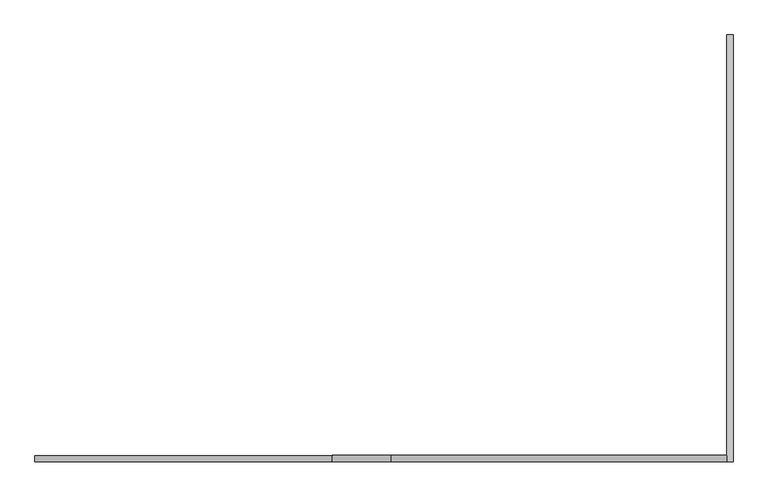
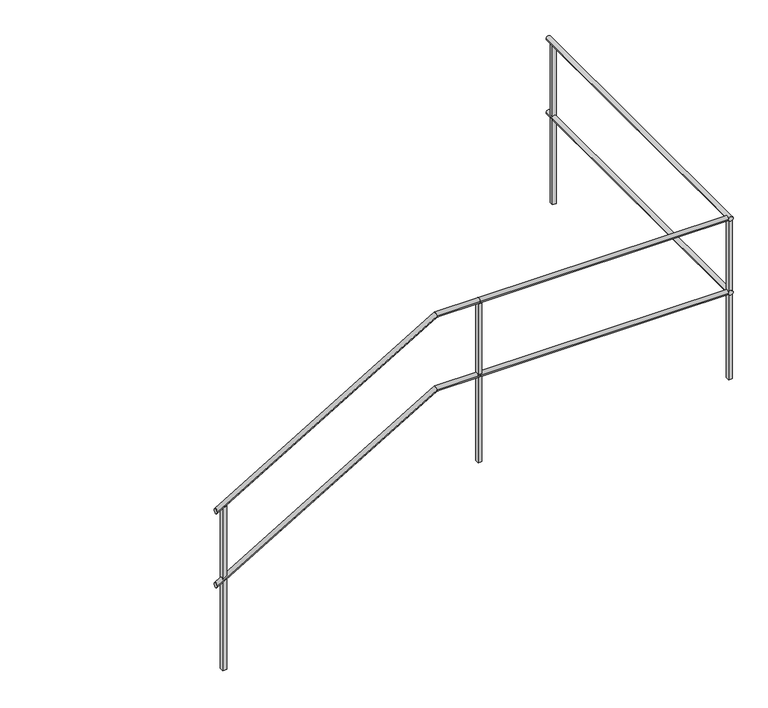
"""IFC4 building model written with IfcOpenShell, lengths in millimetres: railing geometry."""

from ifc_helpers import new_model, si_unit, frame, origin, place, context, project, spatial, polyline, circle_curve, ellipse_curve, outline, extrude, source, transform, mapped, element, save
from ifc_brep_helpers import plane_surface, cylinder_surface, advanced_brep


def railing_42641741(model_context):
    return source(origin(), model_context, "Body", "SolidModel", [
        advanced_brep(
        [(35195.0, -1335.0791411, 749.1723166), (35195.0, -1365.0791411, 749.1723166), (36599.1264386, -1335.0791411, 1584.9618634), (36599.1264386, -1365.0791411, 1584.9618634), (36875.0, -1335.0791411, 1584.9618634), (36875.0, -1365.0791411, 1584.9618634)],
        [
            (0, 1, ellipse_curve(frame((35195.0, -1350.0791411, 749.1723166), z_axis=(-1.0, 0.0, 0.0), x_axis=(0.0, 0.0, -1.0)), 17.4562134, 15.0)),
            (1, 0, ellipse_curve(frame((35195.0, -1350.0791411, 749.1723166), z_axis=(-1.0, 0.0, 0.0), x_axis=(0.0, 0.0, -1.0)), 17.4562134, 15.0)),
            (0, 2),
            (2, 3, ellipse_curve(frame((36599.1264386, -1350.0791411, 1584.9618634), z_axis=(-0.9641817474962143, 0.0, -0.265242450967311), x_axis=(0.265242450967311, 0.0, -0.9641817474962145)), 15.5572329, 15.0)),
            (3, 1),
            (3, 2, ellipse_curve(frame((36599.1264386, -1350.0791411, 1584.9618634), z_axis=(-0.9641817474962143, 0.0, -0.265242450967311), x_axis=(0.265242450967311, 0.0, -0.9641817474962145)), 15.5572329, 15.0)),
            (4, 5, circle_curve(frame((36875.0, -1350.0791411, 1584.9618634), z_axis=(1.0, 0.0, 0.0), x_axis=(0.0, -1.0, 0.0)), 15.0)),
            (5, 4, circle_curve(frame((36875.0, -1350.0791411, 1584.9618634), z_axis=(1.0, 0.0, 0.0), x_axis=(0.0, -1.0, 0.0)), 15.0)),
            (2, 4),
            (5, 3),
        ],
        [
            plane_surface(frame((35195.0, -1350.0791411, 766.62853), z_axis=(-1.0, 0.0, 0.0), x_axis=(0.0, 1.0, 0.0))),
            cylinder_surface(frame((35202.6722579, -1350.0791411, 753.7391368), z_axis=(-0.8592928844097072, 0.0, -0.5114838597676818), x_axis=(0.0, -1.0, 0.0)), 15.0),
            plane_surface(frame((36875.0, -1350.0791411, 1599.9618634), z_axis=(1.0, 0.0, 0.0), x_axis=(0.0, 1.0, 0.0))),
            cylinder_surface(frame((36595.0, -1350.0791411, 1584.9618634), z_axis=(-1.0, 0.0, 0.0), x_axis=(0.0, -1.0, 0.0)), 15.0),
        ],
        [
            (0, [[1, 2]]),
            (1, [[-1, 3, 4, 5]]),
            (1, [[-2, -5, 6, -3]]),
            (2, [[7, 8]]),
            (3, [[-4, 9, -8, 10]]),
            (3, [[-6, -10, -7, -9]]),
        ],
    ),
        advanced_brep(
        [(36875.0, -1335.0791411, 1584.9618634), (36875.0, -1365.0791411, 1584.9618634), (38459.6, -1335.0791411, 1584.9618634), (38459.6, -1365.0791411, 1584.9618634)],
        [
            (0, 1, circle_curve(frame((36875.0, -1350.0791411, 1584.9618634), z_axis=(-1.0, 0.0, 0.0), x_axis=(0.0, -1.0, 0.0)), 15.0)),
            (1, 0, circle_curve(frame((36875.0, -1350.0791411, 1584.9618634), z_axis=(-1.0, 0.0, 0.0), x_axis=(0.0, -1.0, 0.0)), 15.0)),
            (2, 3, circle_curve(frame((38459.6, -1350.0791411, 1584.9618634), z_axis=(1.0, 0.0, 0.0), x_axis=(0.0, -1.0, 0.0)), 15.0)),
            (3, 2, circle_curve(frame((38459.6, -1350.0791411, 1584.9618634), z_axis=(1.0, 0.0, 0.0), x_axis=(0.0, -1.0, 0.0)), 15.0)),
            (0, 2),
            (3, 1),
        ],
        [
            plane_surface(frame((36875.0, -1350.0791411, 1599.9618634), z_axis=(-1.0, 0.0, 0.0), x_axis=(0.0, 1.0, 0.0))),
            plane_surface(frame((38459.6, -1350.0791411, 1599.9618634), z_axis=(1.0, 0.0, 0.0), x_axis=(0.0, 1.0, 0.0))),
            cylinder_surface(frame((36875.0, -1350.0791411, 1584.9618634), z_axis=(-1.0, 0.0, 0.0), x_axis=(0.0, -1.0, 0.0)), 15.0),
        ],
        [
            (0, [[1, 2]]),
            (1, [[3, 4]]),
            (2, [[-1, 5, -4, 6]]),
            (2, [[-2, -6, -3, -5]]),
        ],
    ),
        advanced_brep(
        [(38459.6, -1365.0791411, 1584.9618634), (38489.6, -1365.0791411, 1584.9618634), (38459.6, 649.5208589, 1584.9618634), (38489.6, 649.5208589, 1584.9618634)],
        [
            (0, 1, circle_curve(frame((38474.6, -1365.0791411, 1584.9618634), z_axis=(0.0, -1.0, 0.0), x_axis=(1.0, 0.0, 0.0)), 15.0)),
            (1, 0, circle_curve(frame((38474.6, -1365.0791411, 1584.9618634), z_axis=(0.0, -1.0, 0.0), x_axis=(1.0, 0.0, 0.0)), 15.0)),
            (2, 3, circle_curve(frame((38474.6, 649.5208589, 1584.9618634), z_axis=(0.0, 1.0, 0.0), x_axis=(1.0, 0.0, 0.0)), 15.0)),
            (3, 2, circle_curve(frame((38474.6, 649.5208589, 1584.9618634), z_axis=(0.0, 1.0, 0.0), x_axis=(1.0, 0.0, 0.0)), 15.0)),
            (0, 2),
            (3, 1),
        ],
        [
            plane_surface(frame((38474.6, -1365.0791411, 1599.9618634), z_axis=(0.0, -1.0, 0.0), x_axis=(0.0, 0.0, 1.0))),
            plane_surface(frame((38474.6, 649.5208589, 1599.9618634), z_axis=(0.0, 1.0, 0.0), x_axis=(0.0, 0.0, 1.0))),
            cylinder_surface(frame((38474.6, -1365.0791411, 1584.9618634), z_axis=(0.0, -1.0, 0.0), x_axis=(1.0, 0.0, 0.0)), 15.0),
        ],
        [
            (0, [[1, 2]]),
            (1, [[3, 4]]),
            (2, [[-1, 5, -4, 6]]),
            (2, [[-2, -6, -3, -5]]),
        ],
    ),
        advanced_brep(
        [(35195.0, -1335.0791411, 1249.1723166), (35195.0, -1365.0791411, 1249.1723166), (36599.1264386, -1335.0791411, 2084.9618634), (36599.1264386, -1365.0791411, 2084.9618634), (36875.0, -1335.0791411, 2084.9618634), (36875.0, -1365.0791411, 2084.9618634)],
        [
            (0, 1, ellipse_curve(frame((35195.0, -1350.0791411, 1249.1723166), z_axis=(-1.0, 0.0, 0.0), x_axis=(0.0, 0.0, -1.0)), 17.4562134, 15.0)),
            (1, 0, ellipse_curve(frame((35195.0, -1350.0791411, 1249.1723166), z_axis=(-1.0, 0.0, 0.0), x_axis=(0.0, 0.0, -1.0)), 17.4562134, 15.0)),
            (0, 2),
            (2, 3, ellipse_curve(frame((36599.1264386, -1350.0791411, 2084.9618634), z_axis=(-0.9641817474962143, 0.0, -0.265242450967311), x_axis=(0.265242450967311, 0.0, -0.9641817474962145)), 15.5572329, 15.0)),
            (3, 1),
            (3, 2, ellipse_curve(frame((36599.1264386, -1350.0791411, 2084.9618634), z_axis=(-0.9641817474962143, 0.0, -0.265242450967311), x_axis=(0.265242450967311, 0.0, -0.9641817474962145)), 15.5572329, 15.0)),
            (4, 5, circle_curve(frame((36875.0, -1350.0791411, 2084.9618634), z_axis=(1.0, 0.0, 0.0), x_axis=(0.0, -1.0, 0.0)), 15.0)),
            (5, 4, circle_curve(frame((36875.0, -1350.0791411, 2084.9618634), z_axis=(1.0, 0.0, 0.0), x_axis=(0.0, -1.0, 0.0)), 15.0)),
            (2, 4),
            (5, 3),
        ],
        [
            plane_surface(frame((35195.0, -1350.0791411, 1266.62853), z_axis=(-1.0, 0.0, 0.0), x_axis=(0.0, 1.0, 0.0))),
            cylinder_surface(frame((35202.6722579, -1350.0791411, 1253.7391368), z_axis=(-0.8592928844097072, 0.0, -0.5114838597676818), x_axis=(0.0, -1.0, 0.0)), 15.0),
            plane_surface(frame((36875.0, -1350.0791411, 2099.9618634), z_axis=(1.0, 0.0, 0.0), x_axis=(0.0, 1.0, 0.0))),
            cylinder_surface(frame((36595.0, -1350.0791411, 2084.9618634), z_axis=(-1.0, 0.0, 0.0), x_axis=(0.0, -1.0, 0.0)), 15.0),
        ],
        [
            (0, [[1, 2]]),
            (1, [[-1, 3, 4, 5]]),
            (1, [[-2, -5, 6, -3]]),
            (2, [[7, 8]]),
            (3, [[-4, 9, -8, 10]]),
            (3, [[-6, -10, -7, -9]]),
        ],
    ),
        advanced_brep(
        [(36875.0, -1335.0791411, 2084.9618634), (36875.0, -1365.0791411, 2084.9618634), (38459.6, -1335.0791411, 2084.9618634), (38459.6, -1365.0791411, 2084.9618634)],
        [
            (0, 1, circle_curve(frame((36875.0, -1350.0791411, 2084.9618634), z_axis=(-1.0, 0.0, 0.0), x_axis=(0.0, -1.0, 0.0)), 15.0)),
            (1, 0, circle_curve(frame((36875.0, -1350.0791411, 2084.9618634), z_axis=(-1.0, 0.0, 0.0), x_axis=(0.0, -1.0, 0.0)), 15.0)),
            (2, 3, circle_curve(frame((38459.6, -1350.0791411, 2084.9618634), z_axis=(1.0, 0.0, 0.0), x_axis=(0.0, -1.0, 0.0)), 15.0)),
            (3, 2, circle_curve(frame((38459.6, -1350.0791411, 2084.9618634), z_axis=(1.0, 0.0, 0.0), x_axis=(0.0, -1.0, 0.0)), 15.0)),
            (0, 2),
            (3, 1),
        ],
        [
            plane_surface(frame((36875.0, -1350.0791411, 2099.9618634), z_axis=(-1.0, 0.0, 0.0), x_axis=(0.0, 1.0, 0.0))),
            plane_surface(frame((38459.6, -1350.0791411, 2099.9618634), z_axis=(1.0, 0.0, 0.0), x_axis=(0.0, 1.0, 0.0))),
            cylinder_surface(frame((36875.0, -1350.0791411, 2084.9618634), z_axis=(-1.0, 0.0, 0.0), x_axis=(0.0, -1.0, 0.0)), 15.0),
        ],
        [
            (0, [[1, 2]]),
            (1, [[3, 4]]),
            (2, [[-1, 5, -4, 6]]),
            (2, [[-2, -6, -3, -5]]),
        ],
    ),
        advanced_brep(
        [(38459.6, -1365.0791411, 2084.9618634), (38489.6, -1365.0791411, 2084.9618634), (38459.6, 649.5208589, 2084.9618634), (38489.6, 649.5208589, 2084.9618634)],
        [
            (0, 1, circle_curve(frame((38474.6, -1365.0791411, 2084.9618634), z_axis=(0.0, -1.0, 0.0), x_axis=(1.0, 0.0, 0.0)), 15.0)),
            (1, 0, circle_curve(frame((38474.6, -1365.0791411, 2084.9618634), z_axis=(0.0, -1.0, 0.0), x_axis=(1.0, 0.0, 0.0)), 15.0)),
            (2, 3, circle_curve(frame((38474.6, 649.5208589, 2084.9618634), z_axis=(0.0, 1.0, 0.0), x_axis=(1.0, 0.0, 0.0)), 15.0)),
            (3, 2, circle_curve(frame((38474.6, 649.5208589, 2084.9618634), z_axis=(0.0, 1.0, 0.0), x_axis=(1.0, 0.0, 0.0)), 15.0)),
            (0, 2),
            (3, 1),
        ],
        [
            plane_surface(frame((38474.6, -1365.0791411, 2099.9618634), z_axis=(0.0, -1.0, 0.0), x_axis=(0.0, 0.0, 1.0))),
            plane_surface(frame((38474.6, 649.5208589, 2099.9618634), z_axis=(0.0, 1.0, 0.0), x_axis=(0.0, 0.0, 1.0))),
            cylinder_surface(frame((38474.6, -1365.0791411, 2084.9618634), z_axis=(0.0, -1.0, 0.0), x_axis=(1.0, 0.0, 0.0)), 15.0),
        ],
        [
            (0, [[1, 2]]),
            (1, [[3, 4]]),
            (2, [[-1, 5, -4, 6]]),
            (2, [[-2, -6, -3, -5]]),
        ],
    ),
        extrude(outline(polyline([(38462.1, -1362.5791411), (38462.1, -1337.5791411), (38487.1, -1337.5791411), (38487.1, -1362.5791411), (38462.1, -1362.5791411)])), frame((0.0, 0.0, 999.9618634), z_axis=(0.0, 0.0, 1.0), x_axis=(1.0, 0.0, 0.0)), (0.0, 0.0, 1.0), 1070.0),
        extrude(outline(polyline([(36862.5, -1362.5791411), (36862.5, -1337.5791411), (36887.5, -1337.5791411), (36887.5, -1362.5791411), (36862.5, -1362.5791411)])), frame((0.0, 0.0, 999.9618634), z_axis=(0.0, 0.0, 1.0), x_axis=(1.0, 0.0, 0.0)), (0.0, 0.0, 1.0), 1070.0),
        extrude(outline(polyline([(38487.1, 587.0208589), (38462.1, 587.0208589), (38462.1, 612.0208589), (38487.1, 612.0208589), (38487.1, 587.0208589)])), frame((0.0, 0.0, 999.9618634), z_axis=(0.0, 0.0, 1.0), x_axis=(1.0, 0.0, 0.0)), (0.0, 0.0, 1.0), 1070.0),
        extrude(outline(polyline([(1258.9499586, 35232.5), (166.62853, 35232.5), (166.62853, 35257.5), (1273.830911, 35257.5), (1258.9499586, 35232.5)])), frame((0.0, -1362.5791411, 0.0), z_axis=(0.0, 1.0, 0.0), x_axis=(0.0, 0.0, 1.0)), (0.0, 0.0, 1.0), 25.0),
    ])


if __name__ == "__main__":
    model = new_model("IFC4")
    model_context = context("Model", 3, world=origin())
    ifc_project = project(units=[si_unit("LENGTHUNIT", "METRE", prefix="MILLI")], contexts=[model_context])
    site = spatial("IfcSite", under=ifc_project)
    building = spatial("IfcBuilding", under=site)
    placement = place(None, origin())
    railing_shape = railing_42641741(model_context)
    element("IfcRailing", 1, at=placement, inside=building, context=model_context, shape_type="MappedRepresentation", body=[
        mapped(railing_shape, transform((0.0, 0.0, 0.0), x_axis=(1.0, 0.0, 0.0), y_axis=(0.0, 1.0, 0.0), z_axis=(0.0, 0.0, 1.0))),
    ])
    save(model, "model.ifc")
